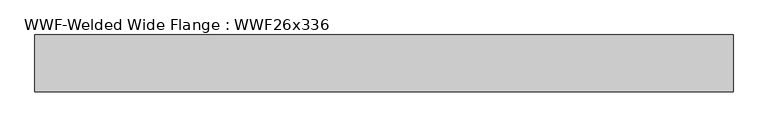
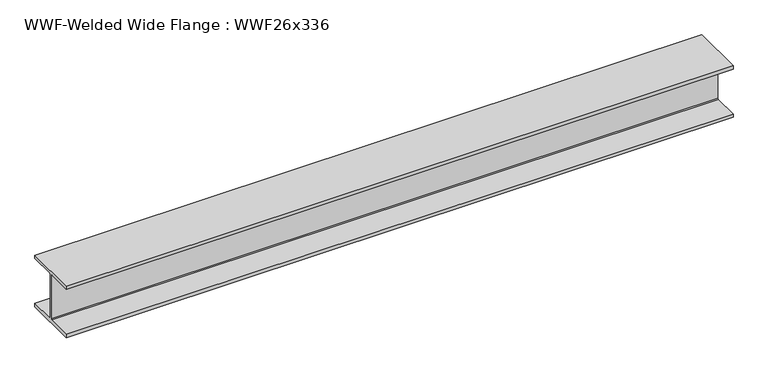
"""IFC4 building model written with IfcOpenShell, lengths in millimetres: beam geometry, WWF-Welded Wide Flange : WWF26x336."""

from ifc_helpers import new_model, si_unit, frame, origin, place, context, project, spatial, polyline, outline, extrude, source, transform, mapped, element, save


def wwf_welded_wide_flange_wwf26x336_96e89ed9(model_context):
    return source(origin(), model_context, "Body", "SweptSolid", [
        extrude(outline(polyline([(324.993, -284.988), (324.993, -324.993), (-324.993, -324.993), (-324.993, -284.988), (-20.6375, -284.988), (-9.9949, -274.3454), (-9.9949, 274.3454), (-20.6375, 284.988), (-324.993, 284.988), (-324.993, 324.993), (324.993, 324.993), (324.993, 284.988), (20.6375, 284.988), (9.9949, 274.3454), (9.9949, -274.3454), (20.6375, -284.988), (324.993, -284.988)])), frame((-3934.8877112, 0.0, 0.0), z_axis=(1.0, 0.0, 0.0), x_axis=(0.0, 1.0, 0.0)), (0.0, 0.0, 1.0), 7999.1298087),
    ])


if __name__ == "__main__":
    model = new_model("IFC4")
    model_context = context("Model", 3, world=origin())
    ifc_project = project(units=[si_unit("LENGTHUNIT", "METRE", prefix="MILLI")], contexts=[model_context])
    site = spatial("IfcSite", under=ifc_project)
    building = spatial("IfcBuilding", under=site)
    placement = place(None, origin())
    wwf_welded_wide_flange_wwf26x336_shape = wwf_welded_wide_flange_wwf26x336_96e89ed9(model_context)
    element("IfcBeam", 1, ObjectType="WWF-Welded Wide Flange : WWF26x336", at=placement, inside=building, context=model_context, shape_type="MappedRepresentation", body=[
        mapped(wwf_welded_wide_flange_wwf26x336_shape, transform((0.0, 0.0, 0.0), x_axis=(1.0, 0.0, 0.0), y_axis=(0.0, 1.0, 0.0), z_axis=(0.0, 0.0, 1.0))),
    ])
    save(model, "model.ifc")

# Revit data of these elements
# Type "WWF-Welded Wide Flange : WWF26x336"
#   Assembly Code = "B10"
#   Nominal d = "12"
#   W = 336
#   Length [instance default] = 1524 mm
#   bf = 649.986 mm
#   d = 649.986 mm
#   k = 20.638 mm
#   tf = 40.005 mm
#   tw = 19.99 mm
#   A = 0.0635483 m²
#   Structural Material [instance default] = Steel ASTM A572
# Element 1 (IfcBeam, "WWF-Welded Wide Flange : WWF26x336")
#   Structural Material = Metal - Steel 43-275
#   Materials on its faces: "Metal - Steel 43-275"
# Materials
#   "Steel ASTM A572": class "Metal", colour RGB 247 247 247, transparency 0, Description = "Structural steel, high strength low alloy, ASTM - A572 - 50", Cost = 0
#   "Metal - Steel 43-275": class "Metal", colour RGB 247 247 247, transparency 0, Cost = 0
